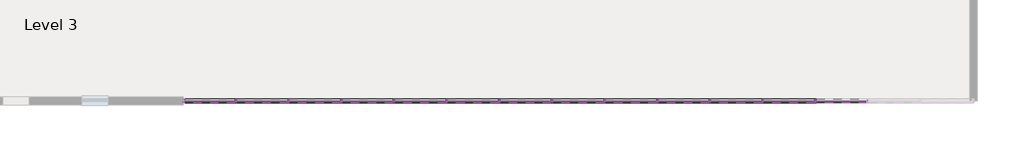
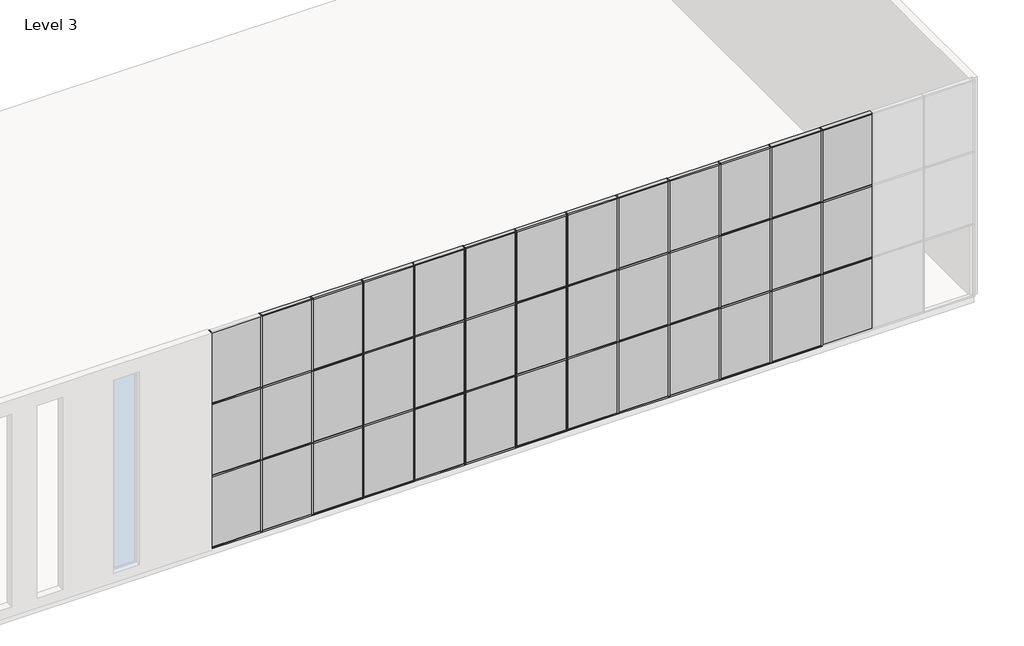
# One storey, part 2 of 4: 87 members, 39 plates.
"""IFC4 building model written with IfcOpenShell, lengths in millimetres."""

import ifcopenshell
import ifcopenshell.guid

model = None  # the IFC model being written
_history = None  # IfcOwnerHistory: only IFC2X3 demands one
_inside = {}  # id of a spatial element -> (the spatial element, [elements in it])
_under = {}  # id of a project, library or spatial element -> (it, [spatial elements below it])
_declared = {}  # id of a project -> (the project, [libraries it declares])
_typed = {}  # id of a type object -> (the type object, [elements of that type])
_made_of = {}  # id of a material, layer set ... -> (it, [elements and type objects made of it])


def new_model(schema):
    """Start an empty IFC model of exactly this schema.

    Asked for "IFC4X3", IfcOpenShell would pick the latest addendum, in which some entities
    have other attributes; the version numbers below select the first issue.
    IFC2X3 requires an IfcOwnerHistory on every rooted entity: one is made here for all.
    """
    global model, _history
    if schema == "IFC4X3":
        model = ifcopenshell.file(schema_version=(4, 3, 0, 0))
    else:
        model = ifcopenshell.file(schema=schema)
    _inside.clear()
    _under.clear()
    _declared.clear()
    _typed.clear()
    _made_of.clear()
    _history = None
    if model.schema == "IFC2X3":
        org = make("IfcOrganization", Name="unknown")
        user = make(
            "IfcPersonAndOrganization",
            ThePerson=make("IfcPerson", FamilyName="unknown"),
            TheOrganization=org,
        )
        app = make(
            "IfcApplication",
            ApplicationDeveloper=org,
            Version="unknown",
            ApplicationFullName="unknown",
            ApplicationIdentifier="unknown",
        )
        _history = make(
            "IfcOwnerHistory",
            OwningUser=user,
            OwningApplication=app,
            ChangeAction="ADDED",
            CreationDate=0,
        )
    return model


def make(cls, **values):
    """One entity of the class cls with the attributes given. An attribute that is None is left unset."""
    return model.create_entity(
        cls, **{name: value for name, value in values.items() if value is not None}
    )


def rooted(cls, **values):
    """An entity with a GlobalId (a new one), such as an element, a storey or a relation."""
    return make(cls, GlobalId=ifcopenshell.guid.new(), OwnerHistory=_history, **values)


def si_unit(unit_type, name, prefix=None):
    """IfcSIUnit, for example si_unit("LENGTHUNIT", "METRE", prefix="MILLI")."""
    return make("IfcSIUnit", UnitType=unit_type, Prefix=prefix, Name=name)


def assignment(units):
    """IfcUnitAssignment: the units of a project."""
    return None if units is None else make("IfcUnitAssignment", Units=units)


def point(xyz):
    """IfcCartesianPoint."""
    return None if xyz is None else make("IfcCartesianPoint", Coordinates=xyz)


def direction(xyz):
    """IfcDirection."""
    return None if xyz is None else make("IfcDirection", DirectionRatios=xyz)


def frame(location, z_axis=None, x_axis=None):
    """IfcAxis2Placement3D, a coordinate frame: its origin and axes. An axis left out is left unset."""
    return make(
        "IfcAxis2Placement3D",
        Location=point(location),
        Axis=direction(z_axis),
        RefDirection=direction(x_axis),
    )


def origin():
    """The frame at (0, 0, 0) with its axes left unset."""
    return frame((0.0, 0.0, 0.0))


def origin_with_axes():
    """The frame at (0, 0, 0) with the z axis (0, 0, 1) and the x axis (1, 0, 0) written out."""
    return frame((0.0, 0.0, 0.0), z_axis=(0.0, 0.0, 1.0), x_axis=(1.0, 0.0, 0.0))


def place(relative_to, where):
    """IfcLocalPlacement: puts the frame where relative to a parent placement (None: the world)."""
    return make(
        "IfcLocalPlacement", PlacementRelTo=relative_to, RelativePlacement=where
    )


def context(
    kind, dimensions, precision=None, world=None, true_north=None, identifier=None
):
    """IfcGeometricRepresentationContext, for example the 3D "Model" context."""
    return make(
        "IfcGeometricRepresentationContext",
        ContextIdentifier=identifier,
        ContextType=kind,
        CoordinateSpaceDimension=dimensions,
        Precision=precision,
        WorldCoordinateSystem=world,
        TrueNorth=true_north,
    )


def project(units=None, contexts=None):
    """IfcProject with its units and contexts."""
    return rooted(
        "IfcProject",
        Name="project",
        RepresentationContexts=contexts,
        UnitsInContext=assignment(units),
    )


def spatial(cls, under=None, at=None, **own):
    """A site, building, storey or space (cls), placed at a placement, below another one or the project."""
    s = rooted(cls, ObjectPlacement=at, **own)
    if under is not None:
        _under.setdefault(under.id(), (under, []))[1].append(s)
    return s


def polyline(points):
    """IfcPolyline through the points."""
    return make("IfcPolyline", Points=[point(p) for p in points])


def outline(outer, holes=None, kind="AREA"):
    """IfcArbitraryClosedProfileDef: a profile drawn as a closed curve; with holes, ...WithVoids."""
    if holes is None:
        return make("IfcArbitraryClosedProfileDef", ProfileType=kind, OuterCurve=outer)
    return make(
        "IfcArbitraryProfileDefWithVoids",
        ProfileType=kind,
        OuterCurve=outer,
        InnerCurves=holes,
    )


def extrude(swept, where, along, depth):
    """IfcExtrudedAreaSolid: the profile swept, set in the frame where, extruded along a direction by depth."""
    return make(
        "IfcExtrudedAreaSolid",
        SweptArea=swept,
        Position=where,
        ExtrudedDirection=direction(along),
        Depth=depth,
    )


def shape(context_of_items, identifier, shape_type, items):
    """IfcShapeRepresentation: the items that make up one representation, for example the "Body"."""
    return make(
        "IfcShapeRepresentation",
        ContextOfItems=context_of_items,
        RepresentationIdentifier=identifier,
        RepresentationType=shape_type,
        Items=items,
    )


def source(mapping_origin, context_of_items, identifier, shape_type, items):
    """IfcRepresentationMap: a shape defined once, which mapped items show again and again."""
    return make(
        "IfcRepresentationMap",
        MappingOrigin=mapping_origin,
        MappedRepresentation=shape(context_of_items, identifier, shape_type, items),
    )


def transform(
    local_origin,
    x_axis=None,
    y_axis=None,
    z_axis=None,
    scale=None,
    scale2=None,
    scale3=None,
    uniform=True,
):
    """IfcCartesianTransformationOperator3D, or its non-uniform kind. x_axis, y_axis, z_axis: its Axis1, 2, 3."""
    if uniform:
        return make(
            "IfcCartesianTransformationOperator3D",
            Axis1=direction(x_axis),
            Axis2=direction(y_axis),
            LocalOrigin=point(local_origin),
            Scale=scale,
            Axis3=direction(z_axis),
        )
    return make(
        "IfcCartesianTransformationOperator3DnonUniform",
        Axis1=direction(x_axis),
        Axis2=direction(y_axis),
        LocalOrigin=point(local_origin),
        Scale=scale,
        Axis3=direction(z_axis),
        Scale2=scale2,
        Scale3=scale3,
    )


def mapped(mapping_source, mapping_target):
    """IfcMappedItem: shows the shape of a source again, moved by a transform."""
    return make(
        "IfcMappedItem", MappingSource=mapping_source, MappingTarget=mapping_target
    )


def made_of(thing, what):
    """Note that an element or type object is made of a material, layer set ...; save() writes the relation."""
    if what is not None:
        _made_of.setdefault(what.id(), (what, []))[1].append(thing)
    return thing


def element(
    cls,
    number,
    at=None,
    inside=None,
    cuts=None,
    type_object=None,
    material=None,
    context=None,
    identifier="Body",
    shape_type=None,
    held_by="IfcProductDefinitionShape",
    body=None,
    shapes=None,
    **own,
):
    """One element of the class cls, such as IfcWall. Its Tag is "e" and its number.

    at: its placement. inside: the storey or other place that contains it. cuts: it is an
    opening in that element (IfcRelVoidsElement). A single representation is given by context,
    identifier, shape_type and body (its items); several are given by shapes. held_by: the class
    of the entity that holds the representations. save() writes the other relations.
    """
    e = rooted(cls, Tag="e%d" % number, ObjectPlacement=at, **own)
    if body is not None:
        shapes = [shape(context, identifier, shape_type, body)]
    if shapes is not None:
        e.Representation = make(held_by, Representations=shapes)
    if inside is not None:
        _inside.setdefault(inside.id(), (inside, []))[1].append(e)
    if cuts is not None:
        rooted(
            "IfcRelVoidsElement", RelatingBuildingElement=cuts, RelatedOpeningElement=e
        )
    if type_object is not None:
        _typed.setdefault(type_object.id(), (type_object, []))[1].append(e)
    return made_of(e, material)


def aggregate(whole, parts):
    """IfcRelAggregates: a whole, such as a stair, and the parts it consists of."""
    return rooted("IfcRelAggregates", RelatingObject=whole, RelatedObjects=parts)


def save(model, path):
    """Write the relations noted so far, then the file.

    IfcRelAggregates (storeys below a building ...), IfcRelContainedInSpatialStructure (elements
    in a storey), IfcRelDefinesByType, IfcRelAssociatesMaterial and IfcRelDeclares: one each for
    every whole, place, type object, material and project.
    """
    for whole, parts in _under.values():
        aggregate(whole, parts)
    for where, things in _inside.values():
        rooted(
            "IfcRelContainedInSpatialStructure",
            RelatedElements=things,
            RelatingStructure=where,
        )
    for kind, things in _typed.values():
        rooted("IfcRelDefinesByType", RelatedObjects=things, RelatingType=kind)
    for what, things in _made_of.values():
        rooted("IfcRelAssociatesMaterial", RelatedObjects=things, RelatingMaterial=what)
    for by, libraries in _declared.values():
        rooted("IfcRelDeclares", RelatingContext=by, RelatedDefinitions=libraries)
    model.write(path)


def rectangular_mullion_50_x_150mm_0967fd3c(model_context):
    return source(origin(), model_context, "Body", "SweptSolid", [
        extrude(outline(polyline([(0.0, 75.0), (0.0, -75.0), (-50.0, -75.0), (-50.0, 75.0), (0.0, 75.0)])), frame((0.0, 0.0, -1950.0000003), z_axis=(0.0, 0.0, 1.0), x_axis=(1.0, 0.0, 0.0)), (0.0, 0.0, 1.0), 1950.0000003),
    ])


def rectangular_mullion_50_x_150mm_f1645b81(model_context):
    return source(origin(), model_context, "Body", "SweptSolid", [
        extrude(outline(polyline([(25.0, 75.0), (25.0, -75.0), (-25.0, -75.0), (-25.0, 75.0), (25.0, 75.0)])), frame((0.0, 0.0, -1950.0000003), z_axis=(0.0, 0.0, 1.0), x_axis=(1.0, 0.0, 0.0)), (0.0, 0.0, 1.0), 1950.0000003),
    ])


def rectangular_mullion_50_x_150mm_6c7cb899(model_context):
    return source(origin(), model_context, "Body", "SweptSolid", [
        extrude(outline(polyline([(25.0, 75.0), (25.0, -75.0), (-25.0, -75.0), (-25.0, 75.0), (25.0, 75.0)])), frame((0.0, 0.0, -3000.0), z_axis=(0.0, 0.0, 1.0), x_axis=(1.0, 0.0, 0.0)), (0.0, 0.0, 1.0), 3000.0),
    ])


def rectangular_mullion_50_x_150mm_d1b252d6(model_context):
    return source(origin(), model_context, "Body", "SweptSolid", [
        extrude(outline(polyline([(0.0, 75.0), (0.0, -75.0), (-50.0, -75.0), (-50.0, 75.0), (0.0, 75.0)])), frame((0.0, 0.0, -1925.0000003), z_axis=(0.0, 0.0, 1.0), x_axis=(1.0, 0.0, 0.0)), (0.0, 0.0, 1.0), 1925.0000003),
    ])


def rectangular_mullion_50_x_150mm_3bfcaf8b(model_context):
    return source(origin(), model_context, "Body", "SweptSolid", [
        extrude(outline(polyline([(25.0, 75.0), (25.0, -75.0), (-25.0, -75.0), (-25.0, 75.0), (25.0, 75.0)])), frame((0.0, 0.0, -1925.0000003), z_axis=(0.0, 0.0, 1.0), x_axis=(1.0, 0.0, 0.0)), (0.0, 0.0, 1.0), 1925.0000003),
    ])


def rectangular_mullion_50_x_150mm_68c91185(model_context):
    return source(origin(), model_context, "Body", "SweptSolid", [
        extrude(outline(polyline([(0.0, 75.0), (0.0, -75.0), (-50.0, -75.0), (-50.0, 75.0), (0.0, 75.0)])), frame((0.0, 0.0, -3000.0), z_axis=(0.0, 0.0, 1.0), x_axis=(1.0, 0.0, 0.0)), (0.0, 0.0, 1.0), 3000.0),
    ])


def system_panel_glazed_156c2b36(model_context):
    return source(origin(), model_context, "Body", "SweptSolid", [
        extrude(outline(polyline([(962.5000001, 24.5), (-962.5000001, 24.5), (-962.5000001, 49.5), (962.5000001, 49.5), (962.5000001, 24.5)])), origin_with_axes(), (0.0, 0.0, 1.0), 2925.0),
    ])


def system_panel_glazed_ecaba6c9(model_context):
    return source(origin(), model_context, "Body", "SweptSolid", [
        extrude(outline(polyline([(975.0, 24.5), (-975.0, 24.5), (-975.0, 49.5), (975.0, 49.5), (975.0, 24.5)])), origin_with_axes(), (0.0, 0.0, 1.0), 2925.0),
    ])


def system_panel_glazed_a9dfd4e8(model_context):
    return source(origin(), model_context, "Body", "SweptSolid", [
        extrude(outline(polyline([(962.5000001, 24.5), (-962.5000001, 24.5), (-962.5000001, 49.5), (962.5000001, 49.5), (962.5000001, 24.5)])), origin_with_axes(), (0.0, 0.0, 1.0), 2950.0),
    ])


def system_panel_glazed_c8490059(model_context):
    return source(origin(), model_context, "Body", "SweptSolid", [
        extrude(outline(polyline([(975.0, 24.5), (-975.0, 24.5), (-975.0, 49.5), (975.0, 49.5), (975.0, 24.5)])), origin_with_axes(), (0.0, 0.0, 1.0), 2950.0),
    ])


model = new_model("IFC4")

# Units and contexts
model_context = context("Model", 3, world=origin())
ifc_project = project(units=[si_unit("LENGTHUNIT", "METRE", prefix="MILLI")], contexts=[model_context])

# Site, building, storey
site = spatial("IfcSite", under=ifc_project)
building = spatial("IfcBuilding", under=site)
storey = spatial("IfcBuildingStorey", under=building, Name="Level 3", Elevation=6000.0)

# Members
placement = place(None, origin())
rectangular_mullion_50_x_150mm_shape = rectangular_mullion_50_x_150mm_0967fd3c(model_context)
element("IfcMember", 1, ObjectType="Rectangular Mullion : 50 x 150mm", at=placement, inside=storey, context=model_context, shape_type="MappedRepresentation", body=[
    mapped(rectangular_mullion_50_x_150mm_shape, transform((12781.4275271, -9138.2971943, 6000.0), x_axis=(0.0, 0.0, -1.0), y_axis=(0.0, 1.0, 0.0), z_axis=(1.0, 0.0, 0.0))),
])
element("IfcMember", 2, ObjectType="Rectangular Mullion : 50 x 150mm", at=placement, inside=storey, context=model_context, shape_type="MappedRepresentation", body=[
    mapped(rectangular_mullion_50_x_150mm_shape, transform((10781.4275272, -9138.2971943, 6000.0), x_axis=(0.0, 0.0, -1.0), y_axis=(0.0, 1.0, 0.0), z_axis=(1.0, 0.0, 0.0))),
])
element("IfcMember", 3, ObjectType="Rectangular Mullion : 50 x 150mm", at=placement, inside=storey, context=model_context, shape_type="MappedRepresentation", body=[
    mapped(rectangular_mullion_50_x_150mm_shape, transform((8781.4275272, -9138.2971943, 6000.0), x_axis=(0.0, 0.0, -1.0), y_axis=(0.0, 1.0, 0.0), z_axis=(1.0, 0.0, 0.0))),
])
element("IfcMember", 4, ObjectType="Rectangular Mullion : 50 x 150mm", at=placement, inside=storey, context=model_context, shape_type="MappedRepresentation", body=[
    mapped(rectangular_mullion_50_x_150mm_shape, transform((6781.4275272, -9138.2971943, 6000.0), x_axis=(0.0, 0.0, -1.0), y_axis=(0.0, 1.0, 0.0), z_axis=(1.0, 0.0, 0.0))),
])
element("IfcMember", 5, ObjectType="Rectangular Mullion : 50 x 150mm", at=placement, inside=storey, context=model_context, shape_type="MappedRepresentation", body=[
    mapped(rectangular_mullion_50_x_150mm_shape, transform((4781.4275273, -9138.2971943, 6000.0), x_axis=(0.0, 0.0, -1.0), y_axis=(0.0, 1.0, 0.0), z_axis=(1.0, 0.0, 0.0))),
])
element("IfcMember", 6, ObjectType="Rectangular Mullion : 50 x 150mm", at=placement, inside=storey, context=model_context, shape_type="MappedRepresentation", body=[
    mapped(rectangular_mullion_50_x_150mm_shape, transform((2781.4275273, -9138.2971943, 6000.0), x_axis=(0.0, 0.0, -1.0), y_axis=(0.0, 1.0, 0.0), z_axis=(1.0, 0.0, 0.0))),
])
element("IfcMember", 7, ObjectType="Rectangular Mullion : 50 x 150mm", at=placement, inside=storey, context=model_context, shape_type="MappedRepresentation", body=[
    mapped(rectangular_mullion_50_x_150mm_shape, transform((781.4275274, -9138.2971943, 6000.0), x_axis=(0.0, 0.0, -1.0), y_axis=(0.0, 1.0, 0.0), z_axis=(1.0, 0.0, 0.0))),
])
element("IfcMember", 8, ObjectType="Rectangular Mullion : 50 x 150mm", at=placement, inside=storey, context=model_context, shape_type="MappedRepresentation", body=[
    mapped(rectangular_mullion_50_x_150mm_shape, transform((-1218.5724726, -9138.2971943, 6000.0), x_axis=(0.0, 0.0, -1.0), y_axis=(0.0, 1.0, 0.0), z_axis=(1.0, 0.0, 0.0))),
])
element("IfcMember", 9, ObjectType="Rectangular Mullion : 50 x 150mm", at=placement, inside=storey, context=model_context, shape_type="MappedRepresentation", body=[
    mapped(rectangular_mullion_50_x_150mm_shape, transform((-3218.5724726, -9138.2971943, 6000.0), x_axis=(0.0, 0.0, -1.0), y_axis=(0.0, 1.0, 0.0), z_axis=(1.0, 0.0, 0.0))),
])
element("IfcMember", 10, ObjectType="Rectangular Mullion : 50 x 150mm", at=placement, inside=storey, context=model_context, shape_type="MappedRepresentation", body=[
    mapped(rectangular_mullion_50_x_150mm_shape, transform((-5218.5724725, -9138.2971943, 6000.0), x_axis=(0.0, 0.0, -1.0), y_axis=(0.0, 1.0, 0.0), z_axis=(1.0, 0.0, 0.0))),
])
element("IfcMember", 11, ObjectType="Rectangular Mullion : 50 x 150mm", at=placement, inside=storey, context=model_context, shape_type="MappedRepresentation", body=[
    mapped(rectangular_mullion_50_x_150mm_shape, transform((-7218.5724725, -9138.2971943, 6000.0), x_axis=(0.0, 0.0, -1.0), y_axis=(0.0, 1.0, 0.0), z_axis=(1.0, 0.0, 0.0))),
])
rectangular_mullion_50_x_150mm_2_shape = rectangular_mullion_50_x_150mm_f1645b81(model_context)
element("IfcMember", 12, ObjectType="Rectangular Mullion : 50 x 150mm", at=placement, inside=storey, context=model_context, shape_type="MappedRepresentation", body=[
    mapped(rectangular_mullion_50_x_150mm_2_shape, transform((12831.4275271, -9138.2971943, 9000.0), x_axis=(0.0, 0.0, 1.0), y_axis=(0.0, 1.0, 0.0), z_axis=(-1.0, 0.0, 0.0))),
])
element("IfcMember", 13, ObjectType="Rectangular Mullion : 50 x 150mm", at=placement, inside=storey, context=model_context, shape_type="MappedRepresentation", body=[
    mapped(rectangular_mullion_50_x_150mm_2_shape, transform((10831.4275272, -9138.2971943, 9000.0), x_axis=(0.0, 0.0, 1.0), y_axis=(0.0, 1.0, 0.0), z_axis=(-1.0, 0.0, 0.0))),
])
element("IfcMember", 14, ObjectType="Rectangular Mullion : 50 x 150mm", at=placement, inside=storey, context=model_context, shape_type="MappedRepresentation", body=[
    mapped(rectangular_mullion_50_x_150mm_2_shape, transform((8831.4275272, -9138.2971943, 9000.0), x_axis=(0.0, 0.0, 1.0), y_axis=(0.0, 1.0, 0.0), z_axis=(-1.0, 0.0, 0.0))),
])
element("IfcMember", 15, ObjectType="Rectangular Mullion : 50 x 150mm", at=placement, inside=storey, context=model_context, shape_type="MappedRepresentation", body=[
    mapped(rectangular_mullion_50_x_150mm_2_shape, transform((6831.4275272, -9138.2971943, 9000.0), x_axis=(0.0, 0.0, 1.0), y_axis=(0.0, 1.0, 0.0), z_axis=(-1.0, 0.0, 0.0))),
])
element("IfcMember", 16, ObjectType="Rectangular Mullion : 50 x 150mm", at=placement, inside=storey, context=model_context, shape_type="MappedRepresentation", body=[
    mapped(rectangular_mullion_50_x_150mm_2_shape, transform((4831.4275273, -9138.2971943, 9000.0), x_axis=(0.0, 0.0, 1.0), y_axis=(0.0, 1.0, 0.0), z_axis=(-1.0, 0.0, 0.0))),
])
element("IfcMember", 17, ObjectType="Rectangular Mullion : 50 x 150mm", at=placement, inside=storey, context=model_context, shape_type="MappedRepresentation", body=[
    mapped(rectangular_mullion_50_x_150mm_2_shape, transform((2831.4275273, -9138.2971943, 9000.0), x_axis=(0.0, 0.0, 1.0), y_axis=(0.0, 1.0, 0.0), z_axis=(-1.0, 0.0, 0.0))),
])
element("IfcMember", 18, ObjectType="Rectangular Mullion : 50 x 150mm", at=placement, inside=storey, context=model_context, shape_type="MappedRepresentation", body=[
    mapped(rectangular_mullion_50_x_150mm_2_shape, transform((831.4275274, -9138.2971943, 9000.0), x_axis=(0.0, 0.0, 1.0), y_axis=(0.0, 1.0, 0.0), z_axis=(-1.0, 0.0, 0.0))),
])
element("IfcMember", 19, ObjectType="Rectangular Mullion : 50 x 150mm", at=placement, inside=storey, context=model_context, shape_type="MappedRepresentation", body=[
    mapped(rectangular_mullion_50_x_150mm_2_shape, transform((-1168.5724726, -9138.2971943, 9000.0), x_axis=(0.0, 0.0, 1.0), y_axis=(0.0, 1.0, 0.0), z_axis=(-1.0, 0.0, 0.0))),
])
element("IfcMember", 20, ObjectType="Rectangular Mullion : 50 x 150mm", at=placement, inside=storey, context=model_context, shape_type="MappedRepresentation", body=[
    mapped(rectangular_mullion_50_x_150mm_2_shape, transform((-3168.5724726, -9138.2971943, 9000.0), x_axis=(0.0, 0.0, 1.0), y_axis=(0.0, 1.0, 0.0), z_axis=(-1.0, 0.0, 0.0))),
])
element("IfcMember", 21, ObjectType="Rectangular Mullion : 50 x 150mm", at=placement, inside=storey, context=model_context, shape_type="MappedRepresentation", body=[
    mapped(rectangular_mullion_50_x_150mm_2_shape, transform((-5168.5724725, -9138.2971943, 9000.0), x_axis=(0.0, 0.0, 1.0), y_axis=(0.0, 1.0, 0.0), z_axis=(-1.0, 0.0, 0.0))),
])
element("IfcMember", 22, ObjectType="Rectangular Mullion : 50 x 150mm", at=placement, inside=storey, context=model_context, shape_type="MappedRepresentation", body=[
    mapped(rectangular_mullion_50_x_150mm_2_shape, transform((-7168.5724725, -9138.2971943, 9000.0), x_axis=(0.0, 0.0, 1.0), y_axis=(0.0, 1.0, 0.0), z_axis=(-1.0, 0.0, 0.0))),
])
element("IfcMember", 23, ObjectType="Rectangular Mullion : 50 x 150mm", at=placement, inside=storey, context=model_context, shape_type="MappedRepresentation", body=[
    mapped(rectangular_mullion_50_x_150mm_2_shape, transform((-9168.5724724, -9138.2971943, 9000.0), x_axis=(0.0, 0.0, 1.0), y_axis=(0.0, 1.0, 0.0), z_axis=(-1.0, 0.0, 0.0))),
])
element("IfcMember", 24, ObjectType="Rectangular Mullion : 50 x 150mm", at=placement, inside=storey, context=model_context, shape_type="MappedRepresentation", body=[
    mapped(rectangular_mullion_50_x_150mm_2_shape, transform((12831.4275271, -9138.2971943, 12000.0), x_axis=(0.0, 0.0, 1.0), y_axis=(0.0, 1.0, 0.0), z_axis=(-1.0, 0.0, 0.0))),
])
element("IfcMember", 25, ObjectType="Rectangular Mullion : 50 x 150mm", at=placement, inside=storey, context=model_context, shape_type="MappedRepresentation", body=[
    mapped(rectangular_mullion_50_x_150mm_2_shape, transform((10831.4275272, -9138.2971943, 12000.0), x_axis=(0.0, 0.0, 1.0), y_axis=(0.0, 1.0, 0.0), z_axis=(-1.0, 0.0, 0.0))),
])
element("IfcMember", 26, ObjectType="Rectangular Mullion : 50 x 150mm", at=placement, inside=storey, context=model_context, shape_type="MappedRepresentation", body=[
    mapped(rectangular_mullion_50_x_150mm_2_shape, transform((8831.4275272, -9138.2971943, 12000.0), x_axis=(0.0, 0.0, 1.0), y_axis=(0.0, 1.0, 0.0), z_axis=(-1.0, 0.0, 0.0))),
])
element("IfcMember", 27, ObjectType="Rectangular Mullion : 50 x 150mm", at=placement, inside=storey, context=model_context, shape_type="MappedRepresentation", body=[
    mapped(rectangular_mullion_50_x_150mm_2_shape, transform((6831.4275272, -9138.2971943, 12000.0), x_axis=(0.0, 0.0, 1.0), y_axis=(0.0, 1.0, 0.0), z_axis=(-1.0, 0.0, 0.0))),
])
element("IfcMember", 28, ObjectType="Rectangular Mullion : 50 x 150mm", at=placement, inside=storey, context=model_context, shape_type="MappedRepresentation", body=[
    mapped(rectangular_mullion_50_x_150mm_2_shape, transform((4831.4275273, -9138.2971943, 12000.0), x_axis=(0.0, 0.0, 1.0), y_axis=(0.0, 1.0, 0.0), z_axis=(-1.0, 0.0, 0.0))),
])
element("IfcMember", 29, ObjectType="Rectangular Mullion : 50 x 150mm", at=placement, inside=storey, context=model_context, shape_type="MappedRepresentation", body=[
    mapped(rectangular_mullion_50_x_150mm_2_shape, transform((2831.4275273, -9138.2971943, 12000.0), x_axis=(0.0, 0.0, 1.0), y_axis=(0.0, 1.0, 0.0), z_axis=(-1.0, 0.0, 0.0))),
])
element("IfcMember", 30, ObjectType="Rectangular Mullion : 50 x 150mm", at=placement, inside=storey, context=model_context, shape_type="MappedRepresentation", body=[
    mapped(rectangular_mullion_50_x_150mm_2_shape, transform((831.4275274, -9138.2971943, 12000.0), x_axis=(0.0, 0.0, 1.0), y_axis=(0.0, 1.0, 0.0), z_axis=(-1.0, 0.0, 0.0))),
])
element("IfcMember", 31, ObjectType="Rectangular Mullion : 50 x 150mm", at=placement, inside=storey, context=model_context, shape_type="MappedRepresentation", body=[
    mapped(rectangular_mullion_50_x_150mm_2_shape, transform((-1168.5724726, -9138.2971943, 12000.0), x_axis=(0.0, 0.0, 1.0), y_axis=(0.0, 1.0, 0.0), z_axis=(-1.0, 0.0, 0.0))),
])
element("IfcMember", 32, ObjectType="Rectangular Mullion : 50 x 150mm", at=placement, inside=storey, context=model_context, shape_type="MappedRepresentation", body=[
    mapped(rectangular_mullion_50_x_150mm_2_shape, transform((-3168.5724726, -9138.2971943, 12000.0), x_axis=(0.0, 0.0, 1.0), y_axis=(0.0, 1.0, 0.0), z_axis=(-1.0, 0.0, 0.0))),
])
element("IfcMember", 33, ObjectType="Rectangular Mullion : 50 x 150mm", at=placement, inside=storey, context=model_context, shape_type="MappedRepresentation", body=[
    mapped(rectangular_mullion_50_x_150mm_2_shape, transform((-5168.5724725, -9138.2971943, 12000.0), x_axis=(0.0, 0.0, 1.0), y_axis=(0.0, 1.0, 0.0), z_axis=(-1.0, 0.0, 0.0))),
])
element("IfcMember", 34, ObjectType="Rectangular Mullion : 50 x 150mm", at=placement, inside=storey, context=model_context, shape_type="MappedRepresentation", body=[
    mapped(rectangular_mullion_50_x_150mm_2_shape, transform((-7168.5724725, -9138.2971943, 12000.0), x_axis=(0.0, 0.0, 1.0), y_axis=(0.0, 1.0, 0.0), z_axis=(-1.0, 0.0, 0.0))),
])
element("IfcMember", 35, ObjectType="Rectangular Mullion : 50 x 150mm", at=placement, inside=storey, context=model_context, shape_type="MappedRepresentation", body=[
    mapped(rectangular_mullion_50_x_150mm_2_shape, transform((-9168.5724724, -9138.2971943, 12000.0), x_axis=(0.0, 0.0, 1.0), y_axis=(0.0, 1.0, 0.0), z_axis=(-1.0, 0.0, 0.0))),
])
element("IfcMember", 36, ObjectType="Rectangular Mullion : 50 x 150mm", at=placement, inside=storey, context=model_context, shape_type="MappedRepresentation", body=[
    mapped(rectangular_mullion_50_x_150mm_shape, transform((12831.4275271, -9138.2971943, 15000.0), x_axis=(0.0, 0.0, 1.0), y_axis=(0.0, 1.0, 0.0), z_axis=(-1.0, 0.0, 0.0))),
])
element("IfcMember", 37, ObjectType="Rectangular Mullion : 50 x 150mm", at=placement, inside=storey, context=model_context, shape_type="MappedRepresentation", body=[
    mapped(rectangular_mullion_50_x_150mm_shape, transform((10831.4275272, -9138.2971943, 15000.0), x_axis=(0.0, 0.0, 1.0), y_axis=(0.0, 1.0, 0.0), z_axis=(-1.0, 0.0, 0.0))),
])
element("IfcMember", 38, ObjectType="Rectangular Mullion : 50 x 150mm", at=placement, inside=storey, context=model_context, shape_type="MappedRepresentation", body=[
    mapped(rectangular_mullion_50_x_150mm_shape, transform((8831.4275272, -9138.2971943, 15000.0), x_axis=(0.0, 0.0, 1.0), y_axis=(0.0, 1.0, 0.0), z_axis=(-1.0, 0.0, 0.0))),
])
element("IfcMember", 39, ObjectType="Rectangular Mullion : 50 x 150mm", at=placement, inside=storey, context=model_context, shape_type="MappedRepresentation", body=[
    mapped(rectangular_mullion_50_x_150mm_shape, transform((6831.4275272, -9138.2971943, 15000.0), x_axis=(0.0, 0.0, 1.0), y_axis=(0.0, 1.0, 0.0), z_axis=(-1.0, 0.0, 0.0))),
])
element("IfcMember", 40, ObjectType="Rectangular Mullion : 50 x 150mm", at=placement, inside=storey, context=model_context, shape_type="MappedRepresentation", body=[
    mapped(rectangular_mullion_50_x_150mm_shape, transform((4831.4275273, -9138.2971943, 15000.0), x_axis=(0.0, 0.0, 1.0), y_axis=(0.0, 1.0, 0.0), z_axis=(-1.0, 0.0, 0.0))),
])
element("IfcMember", 41, ObjectType="Rectangular Mullion : 50 x 150mm", at=placement, inside=storey, context=model_context, shape_type="MappedRepresentation", body=[
    mapped(rectangular_mullion_50_x_150mm_shape, transform((2831.4275273, -9138.2971943, 15000.0), x_axis=(0.0, 0.0, 1.0), y_axis=(0.0, 1.0, 0.0), z_axis=(-1.0, 0.0, 0.0))),
])
element("IfcMember", 42, ObjectType="Rectangular Mullion : 50 x 150mm", at=placement, inside=storey, context=model_context, shape_type="MappedRepresentation", body=[
    mapped(rectangular_mullion_50_x_150mm_shape, transform((831.4275274, -9138.2971943, 15000.0), x_axis=(0.0, 0.0, 1.0), y_axis=(0.0, 1.0, 0.0), z_axis=(-1.0, 0.0, 0.0))),
])
element("IfcMember", 43, ObjectType="Rectangular Mullion : 50 x 150mm", at=placement, inside=storey, context=model_context, shape_type="MappedRepresentation", body=[
    mapped(rectangular_mullion_50_x_150mm_shape, transform((-1168.5724726, -9138.2971943, 15000.0), x_axis=(0.0, 0.0, 1.0), y_axis=(0.0, 1.0, 0.0), z_axis=(-1.0, 0.0, 0.0))),
])
element("IfcMember", 44, ObjectType="Rectangular Mullion : 50 x 150mm", at=placement, inside=storey, context=model_context, shape_type="MappedRepresentation", body=[
    mapped(rectangular_mullion_50_x_150mm_shape, transform((-3168.5724726, -9138.2971943, 15000.0), x_axis=(0.0, 0.0, 1.0), y_axis=(0.0, 1.0, 0.0), z_axis=(-1.0, 0.0, 0.0))),
])
element("IfcMember", 45, ObjectType="Rectangular Mullion : 50 x 150mm", at=placement, inside=storey, context=model_context, shape_type="MappedRepresentation", body=[
    mapped(rectangular_mullion_50_x_150mm_shape, transform((-5168.5724725, -9138.2971943, 15000.0), x_axis=(0.0, 0.0, 1.0), y_axis=(0.0, 1.0, 0.0), z_axis=(-1.0, 0.0, 0.0))),
])
element("IfcMember", 46, ObjectType="Rectangular Mullion : 50 x 150mm", at=placement, inside=storey, context=model_context, shape_type="MappedRepresentation", body=[
    mapped(rectangular_mullion_50_x_150mm_shape, transform((-7168.5724725, -9138.2971943, 15000.0), x_axis=(0.0, 0.0, 1.0), y_axis=(0.0, 1.0, 0.0), z_axis=(-1.0, 0.0, 0.0))),
])
element("IfcMember", 47, ObjectType="Rectangular Mullion : 50 x 150mm", at=placement, inside=storey, context=model_context, shape_type="MappedRepresentation", body=[
    mapped(rectangular_mullion_50_x_150mm_shape, transform((-9168.5724724, -9138.2971943, 15000.0), x_axis=(0.0, 0.0, 1.0), y_axis=(0.0, 1.0, 0.0), z_axis=(-1.0, 0.0, 0.0))),
])
rectangular_mullion_50_x_150mm_3_shape = rectangular_mullion_50_x_150mm_6c7cb899(model_context)
element("IfcMember", 48, ObjectType="Rectangular Mullion : 50 x 150mm", at=placement, inside=storey, context=model_context, shape_type="MappedRepresentation", body=[
    mapped(rectangular_mullion_50_x_150mm_3_shape, transform((12806.4275271, -9138.2971943, 6000.0), x_axis=(-1.0, 0.0, 0.0), y_axis=(0.0, 1.0, 0.0), z_axis=(0.0, 0.0, -1.0))),
])
element("IfcMember", 49, ObjectType="Rectangular Mullion : 50 x 150mm", at=placement, inside=storey, context=model_context, shape_type="MappedRepresentation", body=[
    mapped(rectangular_mullion_50_x_150mm_3_shape, transform((10806.4275272, -9138.2971943, 6000.0), x_axis=(-1.0, 0.0, 0.0), y_axis=(0.0, 1.0, 0.0), z_axis=(0.0, 0.0, -1.0))),
])
element("IfcMember", 50, ObjectType="Rectangular Mullion : 50 x 150mm", at=placement, inside=storey, context=model_context, shape_type="MappedRepresentation", body=[
    mapped(rectangular_mullion_50_x_150mm_3_shape, transform((8806.4275272, -9138.2971943, 6000.0), x_axis=(-1.0, 0.0, 0.0), y_axis=(0.0, 1.0, 0.0), z_axis=(0.0, 0.0, -1.0))),
])
element("IfcMember", 51, ObjectType="Rectangular Mullion : 50 x 150mm", at=placement, inside=storey, context=model_context, shape_type="MappedRepresentation", body=[
    mapped(rectangular_mullion_50_x_150mm_3_shape, transform((6806.4275272, -9138.2971943, 6000.0), x_axis=(-1.0, 0.0, 0.0), y_axis=(0.0, 1.0, 0.0), z_axis=(0.0, 0.0, -1.0))),
])
element("IfcMember", 52, ObjectType="Rectangular Mullion : 50 x 150mm", at=placement, inside=storey, context=model_context, shape_type="MappedRepresentation", body=[
    mapped(rectangular_mullion_50_x_150mm_3_shape, transform((4806.4275273, -9138.2971943, 6000.0), x_axis=(-1.0, 0.0, 0.0), y_axis=(0.0, 1.0, 0.0), z_axis=(0.0, 0.0, -1.0))),
])
element("IfcMember", 53, ObjectType="Rectangular Mullion : 50 x 150mm", at=placement, inside=storey, context=model_context, shape_type="MappedRepresentation", body=[
    mapped(rectangular_mullion_50_x_150mm_3_shape, transform((2806.4275273, -9138.2971943, 6000.0), x_axis=(-1.0, 0.0, 0.0), y_axis=(0.0, 1.0, 0.0), z_axis=(0.0, 0.0, -1.0))),
])
element("IfcMember", 54, ObjectType="Rectangular Mullion : 50 x 150mm", at=placement, inside=storey, context=model_context, shape_type="MappedRepresentation", body=[
    mapped(rectangular_mullion_50_x_150mm_3_shape, transform((806.4275274, -9138.2971943, 6000.0), x_axis=(-1.0, 0.0, 0.0), y_axis=(0.0, 1.0, 0.0), z_axis=(0.0, 0.0, -1.0))),
])
element("IfcMember", 55, ObjectType="Rectangular Mullion : 50 x 150mm", at=placement, inside=storey, context=model_context, shape_type="MappedRepresentation", body=[
    mapped(rectangular_mullion_50_x_150mm_3_shape, transform((-1193.5724726, -9138.2971943, 6000.0), x_axis=(-1.0, 0.0, 0.0), y_axis=(0.0, 1.0, 0.0), z_axis=(0.0, 0.0, -1.0))),
])
element("IfcMember", 56, ObjectType="Rectangular Mullion : 50 x 150mm", at=placement, inside=storey, context=model_context, shape_type="MappedRepresentation", body=[
    mapped(rectangular_mullion_50_x_150mm_3_shape, transform((-3193.5724726, -9138.2971943, 6000.0), x_axis=(-1.0, 0.0, 0.0), y_axis=(0.0, 1.0, 0.0), z_axis=(0.0, 0.0, -1.0))),
])
element("IfcMember", 57, ObjectType="Rectangular Mullion : 50 x 150mm", at=placement, inside=storey, context=model_context, shape_type="MappedRepresentation", body=[
    mapped(rectangular_mullion_50_x_150mm_3_shape, transform((-5193.5724725, -9138.2971943, 6000.0), x_axis=(-1.0, 0.0, 0.0), y_axis=(0.0, 1.0, 0.0), z_axis=(0.0, 0.0, -1.0))),
])
element("IfcMember", 58, ObjectType="Rectangular Mullion : 50 x 150mm", at=placement, inside=storey, context=model_context, shape_type="MappedRepresentation", body=[
    mapped(rectangular_mullion_50_x_150mm_3_shape, transform((-7193.5724725, -9138.2971943, 6000.0), x_axis=(-1.0, 0.0, 0.0), y_axis=(0.0, 1.0, 0.0), z_axis=(0.0, 0.0, -1.0))),
])
element("IfcMember", 59, ObjectType="Rectangular Mullion : 50 x 150mm", at=placement, inside=storey, context=model_context, shape_type="MappedRepresentation", body=[
    mapped(rectangular_mullion_50_x_150mm_3_shape, transform((-9193.5724724, -9138.2971943, 6000.0), x_axis=(-1.0, 0.0, 0.0), y_axis=(0.0, 1.0, 0.0), z_axis=(0.0, 0.0, -1.0))),
])
rectangular_mullion_50_x_150mm_4_shape = rectangular_mullion_50_x_150mm_d1b252d6(model_context)
element("IfcMember", 60, ObjectType="Rectangular Mullion : 50 x 150mm", at=placement, inside=storey, context=model_context, shape_type="MappedRepresentation", body=[
    mapped(rectangular_mullion_50_x_150mm_4_shape, transform((-9218.5724724, -9138.2971943, 6000.0), x_axis=(0.0, 0.0, -1.0), y_axis=(0.0, 1.0, 0.0), z_axis=(1.0, 0.0, 0.0))),
])
rectangular_mullion_50_x_150mm_5_shape = rectangular_mullion_50_x_150mm_3bfcaf8b(model_context)
element("IfcMember", 61, ObjectType="Rectangular Mullion : 50 x 150mm", at=placement, inside=storey, context=model_context, shape_type="MappedRepresentation", body=[
    mapped(rectangular_mullion_50_x_150mm_5_shape, transform((-11143.5724727, -9138.2971943, 9000.0), x_axis=(0.0, 0.0, 1.0), y_axis=(0.0, 1.0, 0.0), z_axis=(-1.0, 0.0, 0.0))),
])
element("IfcMember", 62, ObjectType="Rectangular Mullion : 50 x 150mm", at=placement, inside=storey, context=model_context, shape_type="MappedRepresentation", body=[
    mapped(rectangular_mullion_50_x_150mm_5_shape, transform((-11143.5724727, -9138.2971943, 12000.0), x_axis=(0.0, 0.0, 1.0), y_axis=(0.0, 1.0, 0.0), z_axis=(-1.0, 0.0, 0.0))),
])
element("IfcMember", 63, ObjectType="Rectangular Mullion : 50 x 150mm", at=placement, inside=storey, context=model_context, shape_type="MappedRepresentation", body=[
    mapped(rectangular_mullion_50_x_150mm_3_shape, transform((12806.4275271, -9138.2971943, 9000.0), x_axis=(-1.0, 0.0, 0.0), y_axis=(0.0, 1.0, 0.0), z_axis=(0.0, 0.0, -1.0))),
])
element("IfcMember", 64, ObjectType="Rectangular Mullion : 50 x 150mm", at=placement, inside=storey, context=model_context, shape_type="MappedRepresentation", body=[
    mapped(rectangular_mullion_50_x_150mm_3_shape, transform((10806.4275272, -9138.2971943, 9000.0), x_axis=(-1.0, 0.0, 0.0), y_axis=(0.0, 1.0, 0.0), z_axis=(0.0, 0.0, -1.0))),
])
element("IfcMember", 65, ObjectType="Rectangular Mullion : 50 x 150mm", at=placement, inside=storey, context=model_context, shape_type="MappedRepresentation", body=[
    mapped(rectangular_mullion_50_x_150mm_3_shape, transform((8806.4275272, -9138.2971943, 9000.0), x_axis=(-1.0, 0.0, 0.0), y_axis=(0.0, 1.0, 0.0), z_axis=(0.0, 0.0, -1.0))),
])
element("IfcMember", 66, ObjectType="Rectangular Mullion : 50 x 150mm", at=placement, inside=storey, context=model_context, shape_type="MappedRepresentation", body=[
    mapped(rectangular_mullion_50_x_150mm_3_shape, transform((6806.4275272, -9138.2971943, 9000.0), x_axis=(-1.0, 0.0, 0.0), y_axis=(0.0, 1.0, 0.0), z_axis=(0.0, 0.0, -1.0))),
])
element("IfcMember", 67, ObjectType="Rectangular Mullion : 50 x 150mm", at=placement, inside=storey, context=model_context, shape_type="MappedRepresentation", body=[
    mapped(rectangular_mullion_50_x_150mm_3_shape, transform((4806.4275273, -9138.2971943, 9000.0), x_axis=(-1.0, 0.0, 0.0), y_axis=(0.0, 1.0, 0.0), z_axis=(0.0, 0.0, -1.0))),
])
element("IfcMember", 68, ObjectType="Rectangular Mullion : 50 x 150mm", at=placement, inside=storey, context=model_context, shape_type="MappedRepresentation", body=[
    mapped(rectangular_mullion_50_x_150mm_3_shape, transform((2806.4275273, -9138.2971943, 9000.0), x_axis=(-1.0, 0.0, 0.0), y_axis=(0.0, 1.0, 0.0), z_axis=(0.0, 0.0, -1.0))),
])
element("IfcMember", 69, ObjectType="Rectangular Mullion : 50 x 150mm", at=placement, inside=storey, context=model_context, shape_type="MappedRepresentation", body=[
    mapped(rectangular_mullion_50_x_150mm_3_shape, transform((806.4275274, -9138.2971943, 9000.0), x_axis=(-1.0, 0.0, 0.0), y_axis=(0.0, 1.0, 0.0), z_axis=(0.0, 0.0, -1.0))),
])
element("IfcMember", 70, ObjectType="Rectangular Mullion : 50 x 150mm", at=placement, inside=storey, context=model_context, shape_type="MappedRepresentation", body=[
    mapped(rectangular_mullion_50_x_150mm_3_shape, transform((-1193.5724726, -9138.2971943, 9000.0), x_axis=(-1.0, 0.0, 0.0), y_axis=(0.0, 1.0, 0.0), z_axis=(0.0, 0.0, -1.0))),
])
element("IfcMember", 71, ObjectType="Rectangular Mullion : 50 x 150mm", at=placement, inside=storey, context=model_context, shape_type="MappedRepresentation", body=[
    mapped(rectangular_mullion_50_x_150mm_3_shape, transform((-3193.5724726, -9138.2971943, 9000.0), x_axis=(-1.0, 0.0, 0.0), y_axis=(0.0, 1.0, 0.0), z_axis=(0.0, 0.0, -1.0))),
])
element("IfcMember", 72, ObjectType="Rectangular Mullion : 50 x 150mm", at=placement, inside=storey, context=model_context, shape_type="MappedRepresentation", body=[
    mapped(rectangular_mullion_50_x_150mm_3_shape, transform((-5193.5724725, -9138.2971943, 9000.0), x_axis=(-1.0, 0.0, 0.0), y_axis=(0.0, 1.0, 0.0), z_axis=(0.0, 0.0, -1.0))),
])
element("IfcMember", 73, ObjectType="Rectangular Mullion : 50 x 150mm", at=placement, inside=storey, context=model_context, shape_type="MappedRepresentation", body=[
    mapped(rectangular_mullion_50_x_150mm_3_shape, transform((-7193.5724725, -9138.2971943, 9000.0), x_axis=(-1.0, 0.0, 0.0), y_axis=(0.0, 1.0, 0.0), z_axis=(0.0, 0.0, -1.0))),
])
element("IfcMember", 74, ObjectType="Rectangular Mullion : 50 x 150mm", at=placement, inside=storey, context=model_context, shape_type="MappedRepresentation", body=[
    mapped(rectangular_mullion_50_x_150mm_3_shape, transform((-9193.5724724, -9138.2971943, 9000.0), x_axis=(-1.0, 0.0, 0.0), y_axis=(0.0, 1.0, 0.0), z_axis=(0.0, 0.0, -1.0))),
])
element("IfcMember", 75, ObjectType="Rectangular Mullion : 50 x 150mm", at=placement, inside=storey, context=model_context, shape_type="MappedRepresentation", body=[
    mapped(rectangular_mullion_50_x_150mm_3_shape, transform((12806.4275271, -9138.2971943, 12000.0), x_axis=(-1.0, 0.0, 0.0), y_axis=(0.0, 1.0, 0.0), z_axis=(0.0, 0.0, -1.0))),
])
element("IfcMember", 76, ObjectType="Rectangular Mullion : 50 x 150mm", at=placement, inside=storey, context=model_context, shape_type="MappedRepresentation", body=[
    mapped(rectangular_mullion_50_x_150mm_3_shape, transform((10806.4275272, -9138.2971943, 12000.0), x_axis=(-1.0, 0.0, 0.0), y_axis=(0.0, 1.0, 0.0), z_axis=(0.0, 0.0, -1.0))),
])
element("IfcMember", 77, ObjectType="Rectangular Mullion : 50 x 150mm", at=placement, inside=storey, context=model_context, shape_type="MappedRepresentation", body=[
    mapped(rectangular_mullion_50_x_150mm_3_shape, transform((8806.4275272, -9138.2971943, 12000.0), x_axis=(-1.0, 0.0, 0.0), y_axis=(0.0, 1.0, 0.0), z_axis=(0.0, 0.0, -1.0))),
])
element("IfcMember", 78, ObjectType="Rectangular Mullion : 50 x 150mm", at=placement, inside=storey, context=model_context, shape_type="MappedRepresentation", body=[
    mapped(rectangular_mullion_50_x_150mm_3_shape, transform((6806.4275272, -9138.2971943, 12000.0), x_axis=(-1.0, 0.0, 0.0), y_axis=(0.0, 1.0, 0.0), z_axis=(0.0, 0.0, -1.0))),
])
element("IfcMember", 79, ObjectType="Rectangular Mullion : 50 x 150mm", at=placement, inside=storey, context=model_context, shape_type="MappedRepresentation", body=[
    mapped(rectangular_mullion_50_x_150mm_3_shape, transform((4806.4275273, -9138.2971943, 12000.0), x_axis=(-1.0, 0.0, 0.0), y_axis=(0.0, 1.0, 0.0), z_axis=(0.0, 0.0, -1.0))),
])
element("IfcMember", 80, ObjectType="Rectangular Mullion : 50 x 150mm", at=placement, inside=storey, context=model_context, shape_type="MappedRepresentation", body=[
    mapped(rectangular_mullion_50_x_150mm_3_shape, transform((2806.4275273, -9138.2971943, 12000.0), x_axis=(-1.0, 0.0, 0.0), y_axis=(0.0, 1.0, 0.0), z_axis=(0.0, 0.0, -1.0))),
])
element("IfcMember", 81, ObjectType="Rectangular Mullion : 50 x 150mm", at=placement, inside=storey, context=model_context, shape_type="MappedRepresentation", body=[
    mapped(rectangular_mullion_50_x_150mm_3_shape, transform((806.4275274, -9138.2971943, 12000.0), x_axis=(-1.0, 0.0, 0.0), y_axis=(0.0, 1.0, 0.0), z_axis=(0.0, 0.0, -1.0))),
])
element("IfcMember", 82, ObjectType="Rectangular Mullion : 50 x 150mm", at=placement, inside=storey, context=model_context, shape_type="MappedRepresentation", body=[
    mapped(rectangular_mullion_50_x_150mm_3_shape, transform((-1193.5724726, -9138.2971943, 12000.0), x_axis=(-1.0, 0.0, 0.0), y_axis=(0.0, 1.0, 0.0), z_axis=(0.0, 0.0, -1.0))),
])
element("IfcMember", 83, ObjectType="Rectangular Mullion : 50 x 150mm", at=placement, inside=storey, context=model_context, shape_type="MappedRepresentation", body=[
    mapped(rectangular_mullion_50_x_150mm_3_shape, transform((-3193.5724726, -9138.2971943, 12000.0), x_axis=(-1.0, 0.0, 0.0), y_axis=(0.0, 1.0, 0.0), z_axis=(0.0, 0.0, -1.0))),
])
element("IfcMember", 84, ObjectType="Rectangular Mullion : 50 x 150mm", at=placement, inside=storey, context=model_context, shape_type="MappedRepresentation", body=[
    mapped(rectangular_mullion_50_x_150mm_3_shape, transform((-5193.5724725, -9138.2971943, 12000.0), x_axis=(-1.0, 0.0, 0.0), y_axis=(0.0, 1.0, 0.0), z_axis=(0.0, 0.0, -1.0))),
])
element("IfcMember", 85, ObjectType="Rectangular Mullion : 50 x 150mm", at=placement, inside=storey, context=model_context, shape_type="MappedRepresentation", body=[
    mapped(rectangular_mullion_50_x_150mm_3_shape, transform((-7193.5724725, -9138.2971943, 12000.0), x_axis=(-1.0, 0.0, 0.0), y_axis=(0.0, 1.0, 0.0), z_axis=(0.0, 0.0, -1.0))),
])
element("IfcMember", 86, ObjectType="Rectangular Mullion : 50 x 150mm", at=placement, inside=storey, context=model_context, shape_type="MappedRepresentation", body=[
    mapped(rectangular_mullion_50_x_150mm_3_shape, transform((-9193.5724724, -9138.2971943, 12000.0), x_axis=(-1.0, 0.0, 0.0), y_axis=(0.0, 1.0, 0.0), z_axis=(0.0, 0.0, -1.0))),
])
rectangular_mullion_50_x_150mm_6_shape = rectangular_mullion_50_x_150mm_68c91185(model_context)
element("IfcMember", 87, ObjectType="Rectangular Mullion : 50 x 150mm", at=placement, inside=storey, context=model_context, shape_type="MappedRepresentation", body=[
    mapped(rectangular_mullion_50_x_150mm_6_shape, transform((-11193.5724727, -9138.2971943, 12000.0), x_axis=(-1.0, 0.0, 0.0), y_axis=(0.0, 1.0, 0.0), z_axis=(0.0, 0.0, -1.0))),
])

# Plates
system_panel_glazed_shape = system_panel_glazed_156c2b36(model_context)
element("IfcPlate", 88, ObjectType="System Panel : Glazed", at=placement, inside=storey, context=model_context, shape_type="MappedRepresentation", body=[
    mapped(system_panel_glazed_shape, transform((-10181.0724726, -9138.2971943, 6050.0), x_axis=(-1.0, 0.0, 0.0), y_axis=(0.0, -1.0, 0.0), z_axis=(0.0, 0.0, 1.0))),
])
element("IfcPlate", 89, ObjectType="System Panel : Glazed", at=placement, inside=storey, context=model_context, shape_type="MappedRepresentation", body=[
    mapped(system_panel_glazed_shape, transform((-10181.0724726, -9138.2971943, 12025.0), x_axis=(-1.0, 0.0, 0.0), y_axis=(0.0, -1.0, 0.0), z_axis=(0.0, 0.0, 1.0))),
])
system_panel_glazed_2_shape = system_panel_glazed_ecaba6c9(model_context)
element("IfcPlate", 90, ObjectType="System Panel : Glazed", at=placement, inside=storey, context=model_context, shape_type="MappedRepresentation", body=[
    mapped(system_panel_glazed_2_shape, transform((13806.4275271, -9138.2971943, 6050.0), x_axis=(-1.0, 0.0, 0.0), y_axis=(0.0, -1.0, 0.0), z_axis=(0.0, 0.0, 1.0))),
])
element("IfcPlate", 91, ObjectType="System Panel : Glazed", at=placement, inside=storey, context=model_context, shape_type="MappedRepresentation", body=[
    mapped(system_panel_glazed_2_shape, transform((11806.4275271, -9138.2971943, 6050.0), x_axis=(-1.0, 0.0, 0.0), y_axis=(0.0, -1.0, 0.0), z_axis=(0.0, 0.0, 1.0))),
])
element("IfcPlate", 92, ObjectType="System Panel : Glazed", at=placement, inside=storey, context=model_context, shape_type="MappedRepresentation", body=[
    mapped(system_panel_glazed_2_shape, transform((9806.4275272, -9138.2971943, 6050.0), x_axis=(-1.0, 0.0, 0.0), y_axis=(0.0, -1.0, 0.0), z_axis=(0.0, 0.0, 1.0))),
])
element("IfcPlate", 93, ObjectType="System Panel : Glazed", at=placement, inside=storey, context=model_context, shape_type="MappedRepresentation", body=[
    mapped(system_panel_glazed_2_shape, transform((7806.4275272, -9138.2971943, 6050.0), x_axis=(-1.0, 0.0, 0.0), y_axis=(0.0, -1.0, 0.0), z_axis=(0.0, 0.0, 1.0))),
])
element("IfcPlate", 94, ObjectType="System Panel : Glazed", at=placement, inside=storey, context=model_context, shape_type="MappedRepresentation", body=[
    mapped(system_panel_glazed_2_shape, transform((5806.4275273, -9138.2971943, 6050.0), x_axis=(-1.0, 0.0, 0.0), y_axis=(0.0, -1.0, 0.0), z_axis=(0.0, 0.0, 1.0))),
])
element("IfcPlate", 95, ObjectType="System Panel : Glazed", at=placement, inside=storey, context=model_context, shape_type="MappedRepresentation", body=[
    mapped(system_panel_glazed_2_shape, transform((3806.4275273, -9138.2971943, 6050.0), x_axis=(-1.0, 0.0, 0.0), y_axis=(0.0, -1.0, 0.0), z_axis=(0.0, 0.0, 1.0))),
])
element("IfcPlate", 96, ObjectType="System Panel : Glazed", at=placement, inside=storey, context=model_context, shape_type="MappedRepresentation", body=[
    mapped(system_panel_glazed_2_shape, transform((1806.4275273, -9138.2971943, 6050.0), x_axis=(-1.0, 0.0, 0.0), y_axis=(0.0, -1.0, 0.0), z_axis=(0.0, 0.0, 1.0))),
])
element("IfcPlate", 97, ObjectType="System Panel : Glazed", at=placement, inside=storey, context=model_context, shape_type="MappedRepresentation", body=[
    mapped(system_panel_glazed_2_shape, transform((-193.5724726, -9138.2971943, 6050.0), x_axis=(-1.0, 0.0, 0.0), y_axis=(0.0, -1.0, 0.0), z_axis=(0.0, 0.0, 1.0))),
])
element("IfcPlate", 98, ObjectType="System Panel : Glazed", at=placement, inside=storey, context=model_context, shape_type="MappedRepresentation", body=[
    mapped(system_panel_glazed_2_shape, transform((-2193.5724726, -9138.2971943, 6050.0), x_axis=(-1.0, 0.0, 0.0), y_axis=(0.0, -1.0, 0.0), z_axis=(0.0, 0.0, 1.0))),
])
element("IfcPlate", 99, ObjectType="System Panel : Glazed", at=placement, inside=storey, context=model_context, shape_type="MappedRepresentation", body=[
    mapped(system_panel_glazed_2_shape, transform((-4193.5724725, -9138.2971943, 6050.0), x_axis=(-1.0, 0.0, 0.0), y_axis=(0.0, -1.0, 0.0), z_axis=(0.0, 0.0, 1.0))),
])
element("IfcPlate", 100, ObjectType="System Panel : Glazed", at=placement, inside=storey, context=model_context, shape_type="MappedRepresentation", body=[
    mapped(system_panel_glazed_2_shape, transform((-6193.5724725, -9138.2971943, 6050.0), x_axis=(-1.0, 0.0, 0.0), y_axis=(0.0, -1.0, 0.0), z_axis=(0.0, 0.0, 1.0))),
])
element("IfcPlate", 101, ObjectType="System Panel : Glazed", at=placement, inside=storey, context=model_context, shape_type="MappedRepresentation", body=[
    mapped(system_panel_glazed_2_shape, transform((-8193.5724725, -9138.2971943, 6050.0), x_axis=(-1.0, 0.0, 0.0), y_axis=(0.0, -1.0, 0.0), z_axis=(0.0, 0.0, 1.0))),
])
element("IfcPlate", 102, ObjectType="System Panel : Glazed", at=placement, inside=storey, context=model_context, shape_type="MappedRepresentation", body=[
    mapped(system_panel_glazed_2_shape, transform((13806.4275271, -9138.2971943, 12025.0), x_axis=(-1.0, 0.0, 0.0), y_axis=(0.0, -1.0, 0.0), z_axis=(0.0, 0.0, 1.0))),
])
element("IfcPlate", 103, ObjectType="System Panel : Glazed", at=placement, inside=storey, context=model_context, shape_type="MappedRepresentation", body=[
    mapped(system_panel_glazed_2_shape, transform((11806.4275271, -9138.2971943, 12025.0), x_axis=(-1.0, 0.0, 0.0), y_axis=(0.0, -1.0, 0.0), z_axis=(0.0, 0.0, 1.0))),
])
element("IfcPlate", 104, ObjectType="System Panel : Glazed", at=placement, inside=storey, context=model_context, shape_type="MappedRepresentation", body=[
    mapped(system_panel_glazed_2_shape, transform((9806.4275272, -9138.2971943, 12025.0), x_axis=(-1.0, 0.0, 0.0), y_axis=(0.0, -1.0, 0.0), z_axis=(0.0, 0.0, 1.0))),
])
element("IfcPlate", 105, ObjectType="System Panel : Glazed", at=placement, inside=storey, context=model_context, shape_type="MappedRepresentation", body=[
    mapped(system_panel_glazed_2_shape, transform((7806.4275272, -9138.2971943, 12025.0), x_axis=(-1.0, 0.0, 0.0), y_axis=(0.0, -1.0, 0.0), z_axis=(0.0, 0.0, 1.0))),
])
element("IfcPlate", 106, ObjectType="System Panel : Glazed", at=placement, inside=storey, context=model_context, shape_type="MappedRepresentation", body=[
    mapped(system_panel_glazed_2_shape, transform((5806.4275273, -9138.2971943, 12025.0), x_axis=(-1.0, 0.0, 0.0), y_axis=(0.0, -1.0, 0.0), z_axis=(0.0, 0.0, 1.0))),
])
element("IfcPlate", 107, ObjectType="System Panel : Glazed", at=placement, inside=storey, context=model_context, shape_type="MappedRepresentation", body=[
    mapped(system_panel_glazed_2_shape, transform((3806.4275273, -9138.2971943, 12025.0), x_axis=(-1.0, 0.0, 0.0), y_axis=(0.0, -1.0, 0.0), z_axis=(0.0, 0.0, 1.0))),
])
element("IfcPlate", 108, ObjectType="System Panel : Glazed", at=placement, inside=storey, context=model_context, shape_type="MappedRepresentation", body=[
    mapped(system_panel_glazed_2_shape, transform((1806.4275273, -9138.2971943, 12025.0), x_axis=(-1.0, 0.0, 0.0), y_axis=(0.0, -1.0, 0.0), z_axis=(0.0, 0.0, 1.0))),
])
element("IfcPlate", 109, ObjectType="System Panel : Glazed", at=placement, inside=storey, context=model_context, shape_type="MappedRepresentation", body=[
    mapped(system_panel_glazed_2_shape, transform((-193.5724726, -9138.2971943, 12025.0), x_axis=(-1.0, 0.0, 0.0), y_axis=(0.0, -1.0, 0.0), z_axis=(0.0, 0.0, 1.0))),
])
element("IfcPlate", 110, ObjectType="System Panel : Glazed", at=placement, inside=storey, context=model_context, shape_type="MappedRepresentation", body=[
    mapped(system_panel_glazed_2_shape, transform((-2193.5724726, -9138.2971943, 12025.0), x_axis=(-1.0, 0.0, 0.0), y_axis=(0.0, -1.0, 0.0), z_axis=(0.0, 0.0, 1.0))),
])
element("IfcPlate", 111, ObjectType="System Panel : Glazed", at=placement, inside=storey, context=model_context, shape_type="MappedRepresentation", body=[
    mapped(system_panel_glazed_2_shape, transform((-4193.5724725, -9138.2971943, 12025.0), x_axis=(-1.0, 0.0, 0.0), y_axis=(0.0, -1.0, 0.0), z_axis=(0.0, 0.0, 1.0))),
])
element("IfcPlate", 112, ObjectType="System Panel : Glazed", at=placement, inside=storey, context=model_context, shape_type="MappedRepresentation", body=[
    mapped(system_panel_glazed_2_shape, transform((-6193.5724725, -9138.2971943, 12025.0), x_axis=(-1.0, 0.0, 0.0), y_axis=(0.0, -1.0, 0.0), z_axis=(0.0, 0.0, 1.0))),
])
element("IfcPlate", 113, ObjectType="System Panel : Glazed", at=placement, inside=storey, context=model_context, shape_type="MappedRepresentation", body=[
    mapped(system_panel_glazed_2_shape, transform((-8193.5724725, -9138.2971943, 12025.0), x_axis=(-1.0, 0.0, 0.0), y_axis=(0.0, -1.0, 0.0), z_axis=(0.0, 0.0, 1.0))),
])
system_panel_glazed_3_shape = system_panel_glazed_a9dfd4e8(model_context)
element("IfcPlate", 114, ObjectType="System Panel : Glazed", at=placement, inside=storey, context=model_context, shape_type="MappedRepresentation", body=[
    mapped(system_panel_glazed_3_shape, transform((-10181.0724726, -9138.2971943, 9025.0), x_axis=(-1.0, 0.0, 0.0), y_axis=(0.0, -1.0, 0.0), z_axis=(0.0, 0.0, 1.0))),
])
system_panel_glazed_4_shape = system_panel_glazed_c8490059(model_context)
element("IfcPlate", 115, ObjectType="System Panel : Glazed", at=placement, inside=storey, context=model_context, shape_type="MappedRepresentation", body=[
    mapped(system_panel_glazed_4_shape, transform((13806.4275271, -9138.2971943, 9025.0), x_axis=(-1.0, 0.0, 0.0), y_axis=(0.0, -1.0, 0.0), z_axis=(0.0, 0.0, 1.0))),
])
element("IfcPlate", 116, ObjectType="System Panel : Glazed", at=placement, inside=storey, context=model_context, shape_type="MappedRepresentation", body=[
    mapped(system_panel_glazed_4_shape, transform((11806.4275271, -9138.2971943, 9025.0), x_axis=(-1.0, 0.0, 0.0), y_axis=(0.0, -1.0, 0.0), z_axis=(0.0, 0.0, 1.0))),
])
element("IfcPlate", 117, ObjectType="System Panel : Glazed", at=placement, inside=storey, context=model_context, shape_type="MappedRepresentation", body=[
    mapped(system_panel_glazed_4_shape, transform((9806.4275272, -9138.2971943, 9025.0), x_axis=(-1.0, 0.0, 0.0), y_axis=(0.0, -1.0, 0.0), z_axis=(0.0, 0.0, 1.0))),
])
element("IfcPlate", 118, ObjectType="System Panel : Glazed", at=placement, inside=storey, context=model_context, shape_type="MappedRepresentation", body=[
    mapped(system_panel_glazed_4_shape, transform((7806.4275272, -9138.2971943, 9025.0), x_axis=(-1.0, 0.0, 0.0), y_axis=(0.0, -1.0, 0.0), z_axis=(0.0, 0.0, 1.0))),
])
element("IfcPlate", 119, ObjectType="System Panel : Glazed", at=placement, inside=storey, context=model_context, shape_type="MappedRepresentation", body=[
    mapped(system_panel_glazed_4_shape, transform((5806.4275273, -9138.2971943, 9025.0), x_axis=(-1.0, 0.0, 0.0), y_axis=(0.0, -1.0, 0.0), z_axis=(0.0, 0.0, 1.0))),
])
element("IfcPlate", 120, ObjectType="System Panel : Glazed", at=placement, inside=storey, context=model_context, shape_type="MappedRepresentation", body=[
    mapped(system_panel_glazed_4_shape, transform((3806.4275273, -9138.2971943, 9025.0), x_axis=(-1.0, 0.0, 0.0), y_axis=(0.0, -1.0, 0.0), z_axis=(0.0, 0.0, 1.0))),
])
element("IfcPlate", 121, ObjectType="System Panel : Glazed", at=placement, inside=storey, context=model_context, shape_type="MappedRepresentation", body=[
    mapped(system_panel_glazed_4_shape, transform((1806.4275273, -9138.2971943, 9025.0), x_axis=(-1.0, 0.0, 0.0), y_axis=(0.0, -1.0, 0.0), z_axis=(0.0, 0.0, 1.0))),
])
element("IfcPlate", 122, ObjectType="System Panel : Glazed", at=placement, inside=storey, context=model_context, shape_type="MappedRepresentation", body=[
    mapped(system_panel_glazed_4_shape, transform((-193.5724726, -9138.2971943, 9025.0), x_axis=(-1.0, 0.0, 0.0), y_axis=(0.0, -1.0, 0.0), z_axis=(0.0, 0.0, 1.0))),
])
element("IfcPlate", 123, ObjectType="System Panel : Glazed", at=placement, inside=storey, context=model_context, shape_type="MappedRepresentation", body=[
    mapped(system_panel_glazed_4_shape, transform((-2193.5724726, -9138.2971943, 9025.0), x_axis=(-1.0, 0.0, 0.0), y_axis=(0.0, -1.0, 0.0), z_axis=(0.0, 0.0, 1.0))),
])
element("IfcPlate", 124, ObjectType="System Panel : Glazed", at=placement, inside=storey, context=model_context, shape_type="MappedRepresentation", body=[
    mapped(system_panel_glazed_4_shape, transform((-4193.5724725, -9138.2971943, 9025.0), x_axis=(-1.0, 0.0, 0.0), y_axis=(0.0, -1.0, 0.0), z_axis=(0.0, 0.0, 1.0))),
])
element("IfcPlate", 125, ObjectType="System Panel : Glazed", at=placement, inside=storey, context=model_context, shape_type="MappedRepresentation", body=[
    mapped(system_panel_glazed_4_shape, transform((-6193.5724725, -9138.2971943, 9025.0), x_axis=(-1.0, 0.0, 0.0), y_axis=(0.0, -1.0, 0.0), z_axis=(0.0, 0.0, 1.0))),
])
element("IfcPlate", 126, ObjectType="System Panel : Glazed", at=placement, inside=storey, context=model_context, shape_type="MappedRepresentation", body=[
    mapped(system_panel_glazed_4_shape, transform((-8193.5724725, -9138.2971943, 9025.0), x_axis=(-1.0, 0.0, 0.0), y_axis=(0.0, -1.0, 0.0), z_axis=(0.0, 0.0, 1.0))),
])

save(model, "model.ifc")

# Revit data of these elements
# Project information
#   Project Issue Date = "Issue Date"
#   Project Status = "Project Status"
#   Client Name = "황윤선"
#   Project Address = "Enter address here"
#   Project Name = "202110547"
#   Project Number = "Project Number"
#   Document GUID = "c2a387e2-990c-40c9-8e77-3791c5d4ece9"
# Grids (mm)
#   "1": line (-24193.572, -14250.39) -> (-24193.572, 21655.351)
#   "2": line (-21193.572, -14250.39) -> (-21193.572, 21655.351)
#   "3": line (-11193.572, -14250.39) -> (-11193.572, 21655.351)
#   "4": line (-1193.572, -14250.39) -> (-1193.572, 21655.351)
#   "5": line (8806.428, -14250.39) -> (8806.428, 21655.351)
#   "6": line (18806.428, -14250.39) -> (18806.428, 21655.351)
#   "A": line (25403.309, 16861.703) -> (-28721.065, 16861.703)
#   "B": line (25403.309, 13861.703) -> (-28721.065, 13861.703)
#   "C": line (25403.309, 3861.703) -> (-28721.065, 3861.703)
#   "D": line (25403.309, -6138.297) -> (-28721.065, -6138.297)
#   "E": line (25403.309, -9138.297) -> (-28721.065, -9138.297)
# Type "Rectangular Mullion : 50 x 150mm"
#   built-in parameter 1007304 = 0.492126 (stored number, unit not read)
#   built-in parameter 1007301 = 0.082021 (stored number, unit not read)
#   built-in parameter 1007300 = 0.082021 (stored number, unit not read)
# Elements 1, 2, 3, 4, 5, 6, 7, 8, 9, 10, 11, 12, 13, 14, 15, 16, 17, 18, 19, 20, 21, 22, 23, 24, 25, 26, 27, 28, 29, 30, 31, 32, 33, 34, 35, 36, 37, 38, 39, 40, 41, 42, 43, 44, 45, 46, 47, 48, 49, 50, 51, 52, 53, 54, 55, 56, 57, 58, 59, 60, 61, 62, 63, 64, 65, 66, 67, 68, 69, 70, 71, 72, 73, 74, 75, 76, 77, 78, 79, 80, 81, 82, 83, 84, 85, 86, 87 (IfcMember, "Rectangular Mullion : 50 x 150mm")
#   Phase Created = New Construction
#   Materials on its faces: "Metal - Aluminium"
# Elements 88, 89, 90, 91, 92, 93, 94, 95, 96, 97, 98, 99, 100, 101, 102, 103, 104, 105, 106, 107, 108, 109, 110, 111, 112, 113, 114, 115, 116, 117, 118, 119, 120, 121, 122, 123, 124, 125, 126 (IfcPlate, "System Panel : Glazed")
#   Phase Created = New Construction
#   Materials on its faces: "Glass"
# Materials
#   "Metal - Aluminium": class "Metal", colour RGB 247 247 247, transparency 0
#   "Glass": class "Glass", colour RGB 0 128 192, transparency 0.9
